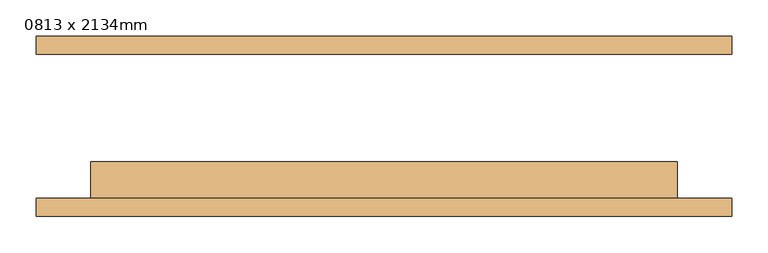
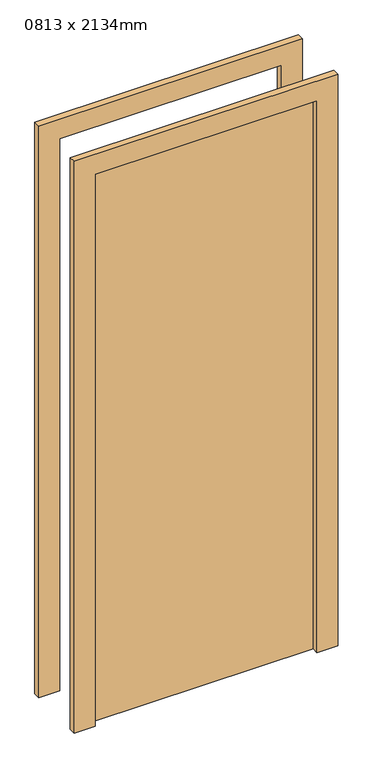
"""IFC4 building model written with IfcOpenShell, lengths in millimetres: door geometry, M_Folha única : 0813 x 2134mm."""

from ifc_helpers import new_model, si_unit, frame, origin, origin_with_axes, place, context, project, spatial, polyline, outline, extrude, source, transform, mapped, element, save


def door_0813_x_2134mm_c8a1819b(model_context):
    return source(origin(), model_context, "Body", "SweptSolid", [
        extrude(outline(polyline([(2210.0, -482.5), (0.0, -482.5), (0.0, -406.5), (2134.0, -406.5), (2134.0, 406.5), (0.0, 406.5), (0.0, 482.5), (2210.0, 482.5), (2210.0, -482.5)])), frame((0.0, -125.0, 0.0), z_axis=(0.0, 1.0, 0.0), x_axis=(0.0, 0.0, 1.0)), (0.0, 0.0, 1.0), 25.0),
        extrude(outline(polyline([(2210.0, 482.5), (2210.0, -482.5), (0.0, -482.5), (0.0, -406.5), (2134.0, -406.5), (2134.0, 406.5), (0.0, 406.5), (0.0, 482.5), (2210.0, 482.5)])), frame((0.0, 100.0, 0.0), z_axis=(0.0, 1.0, 0.0), x_axis=(0.0, 0.0, 1.0)), (0.0, 0.0, 1.0), 25.0),
        extrude(outline(polyline([(406.5, -49.0), (406.5, -100.0), (-406.5, -100.0), (-406.5, -49.0), (406.5, -49.0)])), origin_with_axes(), (0.0, 0.0, 1.0), 2134.0),
    ])


if __name__ == "__main__":
    model = new_model("IFC4")
    model_context = context("Model", 3, world=origin())
    ifc_project = project(units=[si_unit("LENGTHUNIT", "METRE", prefix="MILLI")], contexts=[model_context])
    site = spatial("IfcSite", under=ifc_project)
    building = spatial("IfcBuilding", under=site)
    placement = place(None, origin())
    door_0813_x_2134mm_shape = door_0813_x_2134mm_c8a1819b(model_context)
    element("IfcDoor", 1, ObjectType="M_Folha única : 0813 x 2134mm", at=placement, inside=building, context=model_context, shape_type="MappedRepresentation", body=[
        mapped(door_0813_x_2134mm_shape, transform((0.0, 0.0, 0.0), x_axis=(1.0, 0.0, 0.0), y_axis=(0.0, 1.0, 0.0), z_axis=(0.0, 0.0, 1.0))),
    ])
    save(model, "model.ifc")

# Revit data of these elements
# Type "M_Folha única : 0813 x 2134mm"
#   Type Mark = "24"
#   Construction Type Id = "MDOOR"
#   Analytic Construction = "Metal"
#   Thickness = 0.051 m
#   Thermal Resistance (R) = 0.270117 (m²·K)/W
#   Heat Transfer Coefficient (U) = 3.7021 W/(m²·K)
#   Height = 2.134 m
#   Projeção da apara externa = 0.025 m
#   Projeção da apara interna = 0.025 m
#   Largura da apara = 0.076 m
#   Width = 0.813 m
#   Define Thermal Properties by = 1
#   Define Thermal Properties by = 1
#   Material da porta = Porta - Painel
#   Material da moldura = Porta - Batente
#   Visual Light Transmittance = 0
#   Solar Heat Gain Coefficient = 0
#   Function = (empty or 0)
#   Wall Closure = (empty or 0)
# Element 1 (IfcDoor, "M_Folha única : 0813 x 2134mm")
#   Materials on its faces: "Porta - Batente", "Porta - Painel"
# Materials
#   "Porta - Painel": class "Madeira", colour RGB 210 159 95, transparency 0, Cost = 0
#   "Porta - Batente": class "Diversos", colour RGB 118 70 51, transparency 0, Cost = 0
